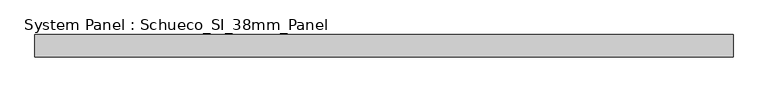
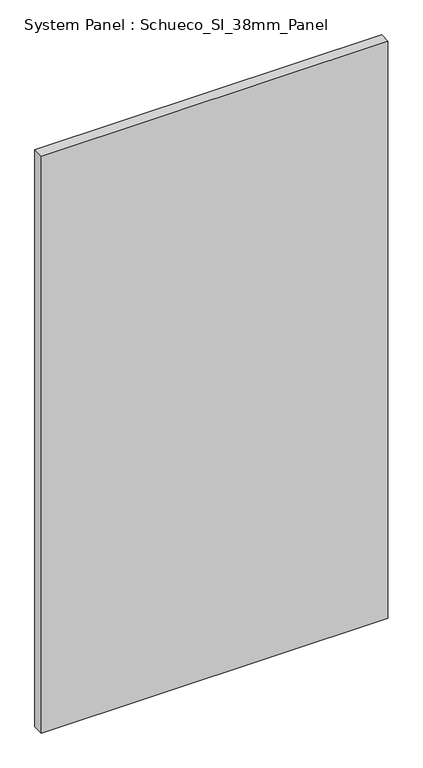
"""IFC4 building model written with IfcOpenShell, lengths in millimetres: plate geometry, System Panel : Schueco_SI_38mm_Panel."""

from ifc_helpers import new_model, si_unit, origin, origin_with_axes, place, context, project, spatial, polyline, outline, extrude, source, transform, mapped, element, save


def system_panel_schueco_si_38mm_panel_01bbaa69(model_context):
    return source(origin(), model_context, "Body", "SweptSolid", [
        extrude(outline(polyline([(599.0, -38.0), (-599.0, -38.0), (-599.0, 0.0), (599.0, 0.0), (599.0, -38.0)])), origin_with_axes(), (0.0, 0.0, 1.0), 2108.0),
    ])


if __name__ == "__main__":
    model = new_model("IFC4")
    model_context = context("Model", 3, world=origin())
    ifc_project = project(units=[si_unit("LENGTHUNIT", "METRE", prefix="MILLI")], contexts=[model_context])
    site = spatial("IfcSite", under=ifc_project)
    building = spatial("IfcBuilding", under=site)
    placement = place(None, origin())
    system_panel_schueco_si_38mm_panel_shape = system_panel_schueco_si_38mm_panel_01bbaa69(model_context)
    element("IfcPlate", 1, ObjectType="System Panel : Schueco_SI_38mm_Panel", at=placement, inside=building, context=model_context, shape_type="MappedRepresentation", body=[
        mapped(system_panel_schueco_si_38mm_panel_shape, transform((0.0, 0.0, 0.0), x_axis=(1.0, 0.0, 0.0), y_axis=(0.0, 1.0, 0.0), z_axis=(0.0, 0.0, 1.0))),
    ])
    save(model, "model.ifc")

# Revit data of these elements
# Type "System Panel : Schueco_SI_38mm_Panel"
#   Model = "Panel 38mm"
# Element 1 (IfcPlate, "System Panel : Schueco_SI_38mm_Panel")
#   Materials on its faces: "Alu"
# Materials
#   "Alu": class "Glas", colour RGB 140 140 140, transparency 0
